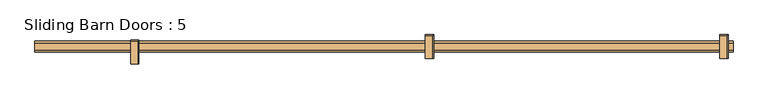
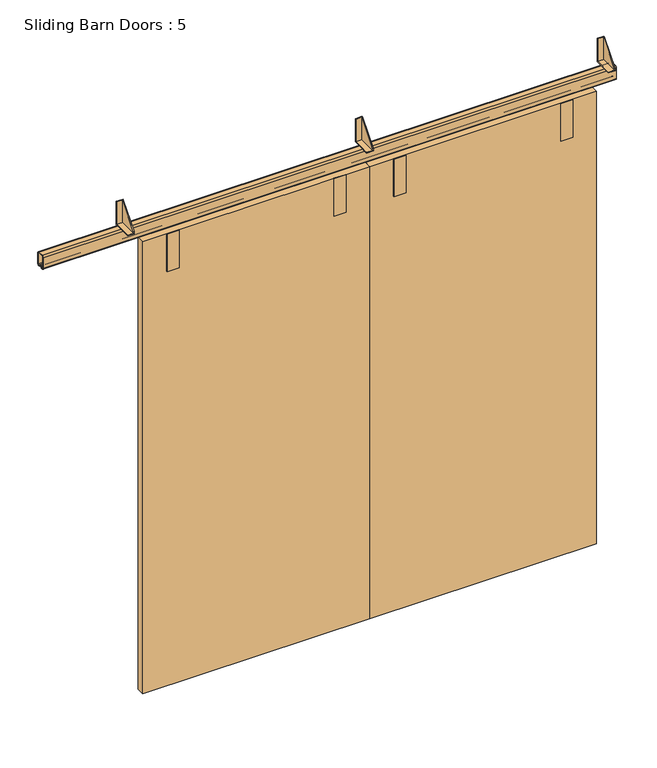
"""IFC4 building model written with IfcOpenShell, lengths in millimetres: door geometry, Sliding Barn Doors : 5."""

from ifc_helpers import new_model, si_unit, point, frame, frame_2d, origin, place, context, project, spatial, polyline, circle_curve, trimmed, segment, composite_curve, outline, extrude, source, transform, mapped, element, save


def sliding_barn_doors_5_394c9385(model_context):
    return source(origin(), model_context, "Body", "SweptSolid", [
        extrude(outline(polyline([(-158.75, 2152.65), (-79.375, 2247.773), (-79.375, 2146.3), (-158.75, 2146.3), (-158.75, 2152.65)])), frame((-1512.9371094, 0.0, 0.0), z_axis=(1.0, 0.0, 0.0), x_axis=(0.0, 1.0, 0.0)), (0.0, 0.0, 1.0), 3.175),
        extrude(outline(polyline([(-76.2, 2143.125), (-158.75, 2143.125), (-158.75, 2146.3), (-79.375, 2146.3), (-79.375, 2247.773), (-76.2, 2247.773), (-76.2, 2143.125)])), frame((-1538.2378906, 0.0, 0.0), z_axis=(1.0, 0.0, 0.0), x_axis=(0.0, 1.0, 0.0)), (0.0, 0.0, 1.0), 28.4757812),
        extrude(outline(polyline([(-139.7, 2152.65), (-60.325, 2247.773), (-60.325, 2146.3), (-139.7, 2146.3), (-139.7, 2152.65)])), frame((-484.2371094, 0.0, 0.0), z_axis=(1.0, 0.0, 0.0), x_axis=(0.0, 1.0, 0.0)), (0.0, 0.0, 1.0), 3.175),
        extrude(outline(polyline([(-57.15, 2143.125), (-139.7, 2143.125), (-139.7, 2146.3), (-60.325, 2146.3), (-60.325, 2247.773), (-57.15, 2247.773), (-57.15, 2143.125)])), frame((-509.5378906, 0.0, 0.0), z_axis=(1.0, 0.0, 0.0), x_axis=(0.0, 1.0, 0.0)), (0.0, 0.0, 1.0), 28.4757813),
        extrude(outline(polyline([(-139.7, 2152.65), (-60.325, 2247.773), (-60.325, 2146.3), (-139.7, 2146.3), (-139.7, 2152.65)])), frame((544.4628906, 0.0, 0.0), z_axis=(1.0, 0.0, 0.0), x_axis=(0.0, 1.0, 0.0)), (0.0, 0.0, 1.0), 3.175),
        extrude(outline(polyline([(-57.15, 2143.125), (-139.7, 2143.125), (-139.7, 2146.3), (-60.325, 2146.3), (-60.325, 2247.773), (-57.15, 2247.773), (-57.15, 2143.125)])), frame((519.1621094, 0.0, 0.0), z_axis=(1.0, 0.0, 0.0), x_axis=(0.0, 1.0, 0.0)), (0.0, 0.0, 1.0), 28.4757813),
        extrude(outline(polyline([(-1346.454, -117.475), (-1346.454, -114.3), (-1295.146, -114.3), (-1295.146, -117.475), (-1346.454, -117.475)])), frame((0.0, 0.0, 1889.252), z_axis=(0.0, 0.0, 1.0), x_axis=(1.0, 0.0, 0.0)), (0.0, 0.0, 1.0), 168.148),
        extrude(outline(polyline([(-635.254, -117.475), (-635.254, -114.3), (-583.946, -114.3), (-583.946, -117.475), (-635.254, -117.475)])), frame((0.0, 0.0, 1889.252), z_axis=(0.0, 0.0, 1.0), x_axis=(1.0, 0.0, 0.0)), (0.0, 0.0, 1.0), 168.148),
        extrude(outline(polyline([(-381.254, -117.475), (-381.254, -114.3), (-329.946, -114.3), (-329.946, -117.475), (-381.254, -117.475)])), frame((0.0, 0.0, 1889.252), z_axis=(0.0, 0.0, 1.0), x_axis=(1.0, 0.0, 0.0)), (0.0, 0.0, 1.0), 168.148),
        extrude(outline(polyline([(329.946, -117.475), (329.946, -114.3), (381.254, -114.3), (381.254, -117.475), (329.946, -117.475)])), frame((0.0, 0.0, 1889.252), z_axis=(0.0, 0.0, 1.0), x_axis=(1.0, 0.0, 0.0)), (0.0, 0.0, 1.0), 168.148),
        extrude(outline(polyline([(-1447.8, -114.3), (-1447.8, -79.375), (-482.6, -79.375), (-482.6, -114.3), (-1447.8, -114.3)])), frame((0.0, 0.0, 25.4), z_axis=(0.0, 0.0, 1.0), x_axis=(1.0, 0.0, 0.0)), (0.0, 0.0, 1.0), 2032.0),
        extrude(outline(polyline([(-482.6, -114.3), (-482.6, -79.375), (482.6, -79.375), (482.6, -114.3), (-482.6, -114.3)])), frame((0.0, 0.0, 25.4), z_axis=(0.0, 0.0, 1.0), x_axis=(1.0, 0.0, 0.0)), (0.0, 0.0, 1.0), 2032.0),
        extrude(outline(composite_curve([segment(trimmed(circle_curve(frame_2d((-85.725, 2136.775)), 6.35), [point((-85.725, 2143.125))], [point((-79.375, 2136.775))], False, "CARTESIAN"), True, "CONTINUOUS"), segment(polyline([(-79.375, 2136.775), (-79.375, 2088.515)]), True, "CONTINUOUS"), segment(trimmed(circle_curve(frame_2d((-85.725, 2088.515)), 6.35), [point((-79.375, 2088.515))], [point((-85.725, 2082.165))], False, "CARTESIAN"), True, "CONTINUOUS"), segment(polyline([(-85.725, 2082.165), (-91.1336853, 2082.165)]), True, "CONTINUOUS"), segment(trimmed(circle_curve(frame_2d((-91.1336853, 2083.7525)), 1.5875), [point((-91.1336853, 2082.165))], [point((-92.6920184, 2083.4495907))], False, "CARTESIAN"), True, "CONTINUOUS"), segment(polyline([(-92.6920184, 2083.4495907), (-94.1175341, 2090.7832331), (-92.6013971, 2090.7832331), (-91.2154749, 2083.6532812), (-85.725, 2083.6532812)]), True, "CONTINUOUS"), segment(trimmed(circle_curve(frame_2d((-85.725, 2088.515)), 4.8617187), [point((-85.725, 2083.6532812))], [point((-80.8632813, 2088.515))], True, "CARTESIAN"), True, "CONTINUOUS"), segment(polyline([(-80.8632813, 2088.515), (-80.8632813, 2136.775)]), True, "CONTINUOUS"), segment(trimmed(circle_curve(frame_2d((-85.725, 2136.775)), 4.8617187), [point((-80.8632813, 2136.775))], [point((-85.725, 2141.6367187))], True, "CARTESIAN"), True, "CONTINUOUS"), segment(polyline([(-85.725, 2141.6367187), (-111.252, 2141.6367187)]), True, "CONTINUOUS"), segment(trimmed(circle_curve(frame_2d((-111.252, 2136.775)), 4.8617187), [point((-111.252, 2141.6367187))], [point((-116.1137188, 2136.775))], True, "CARTESIAN"), True, "CONTINUOUS"), segment(polyline([(-116.1137188, 2136.775), (-116.1137188, 2088.515)]), True, "CONTINUOUS"), segment(trimmed(circle_curve(frame_2d((-111.252, 2088.515)), 4.8617187), [point((-116.1137188, 2088.515))], [point((-111.252, 2083.6532812))], True, "CARTESIAN"), True, "CONTINUOUS"), segment(polyline([(-111.252, 2083.6532812), (-105.7615251, 2083.6532812), (-104.3756029, 2090.7832331), (-102.8594659, 2090.7832331), (-104.2849816, 2083.4495907)]), True, "CONTINUOUS"), segment(trimmed(circle_curve(frame_2d((-105.8433147, 2083.7525)), 1.5875), [point((-104.2849816, 2083.4495907))], [point((-105.8433147, 2082.165))], False, "CARTESIAN"), True, "CONTINUOUS"), segment(polyline([(-105.8433147, 2082.165), (-111.252, 2082.165)]), True, "CONTINUOUS"), segment(trimmed(circle_curve(frame_2d((-111.252, 2088.515)), 6.35), [point((-111.252, 2082.165))], [point((-117.602, 2088.515))], False, "CARTESIAN"), True, "CONTINUOUS"), segment(polyline([(-117.602, 2088.515), (-117.602, 2136.775)]), True, "CONTINUOUS"), segment(trimmed(circle_curve(frame_2d((-111.252, 2136.775)), 6.35), [point((-117.602, 2136.775))], [point((-111.252, 2143.125))], False, "CARTESIAN"), True, "CONTINUOUS"), segment(polyline([(-111.252, 2143.125), (-85.725, 2143.125)]), True, "CONTINUOUS")], self_intersect=False)), frame((-1873.25, 0.0, 0.0), z_axis=(1.0, 0.0, 0.0), x_axis=(0.0, 1.0, 0.0)), (0.0, 0.0, 1.0), 2438.4),
    ])


if __name__ == "__main__":
    model = new_model("IFC4")
    model_context = context("Model", 3, world=origin())
    ifc_project = project(units=[si_unit("LENGTHUNIT", "METRE", prefix="MILLI")], contexts=[model_context])
    site = spatial("IfcSite", under=ifc_project)
    building = spatial("IfcBuilding", under=site)
    placement = place(None, origin())
    sliding_barn_doors_5_shape = sliding_barn_doors_5_394c9385(model_context)
    element("IfcDoor", 1, ObjectType="Sliding Barn Doors : 5", at=placement, inside=building, context=model_context, shape_type="MappedRepresentation", body=[
        mapped(sliding_barn_doors_5_shape, transform((0.0, 0.0, 0.0), x_axis=(1.0, 0.0, 0.0), y_axis=(0.0, 1.0, 0.0), z_axis=(0.0, 0.0, 1.0))),
    ])
    save(model, "model.ifc")

# Revit data of these elements
# Type "Sliding Barn Doors : 5"
#   Type Mark = "46"
#   Analytic Construction = "<None>"
#   rail_overlap_left = 0' - 5 1/4"
#   rail_length = 8' - 0"
#   overlap_left = 0' - 2"
#   overlap = 0' - 0"
#   bracket_right = 3' - 7"
#   bracket_left = 0' - 4"
#   Thickness = 0' - 1 3/8"
#   Panel Width = 3' - 2"
#   Panel Height = 6' - 8"
#   Gap 2 = 0' - 0 1/2"
#   Gap 1 = 0' - 0 7/8"
#   Frame Projection Ext. = 0' - 1"
#   Frame Projection Int. = 0' - 1"
#   Frame Width = 0' - 3"
#   Height = 6' - 4"
#   Width = 2' - 10"
#   Bracket_offset = 0' - 5"
#   Door_4 = no
#   Door_3 = no
#   Hardware Material = Metal - Aluminum
#   Door Material = Closet_1
#   Function = (empty or 0)
#   Wall Closure = (empty or 0)
# Element 1 (IfcDoor, "Sliding Barn Doors : 5")
#   Materials on its faces: "Metal - Aluminum", "Closet_1"
# Materials
#   "Metal - Aluminum": class "Metal", colour RGB 247 247 247, transparency 0
#   "Closet_1": class "Paint", colour RGB 58 62 47, transparency 0, Cost = 0
